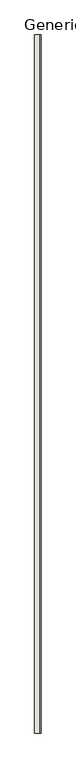
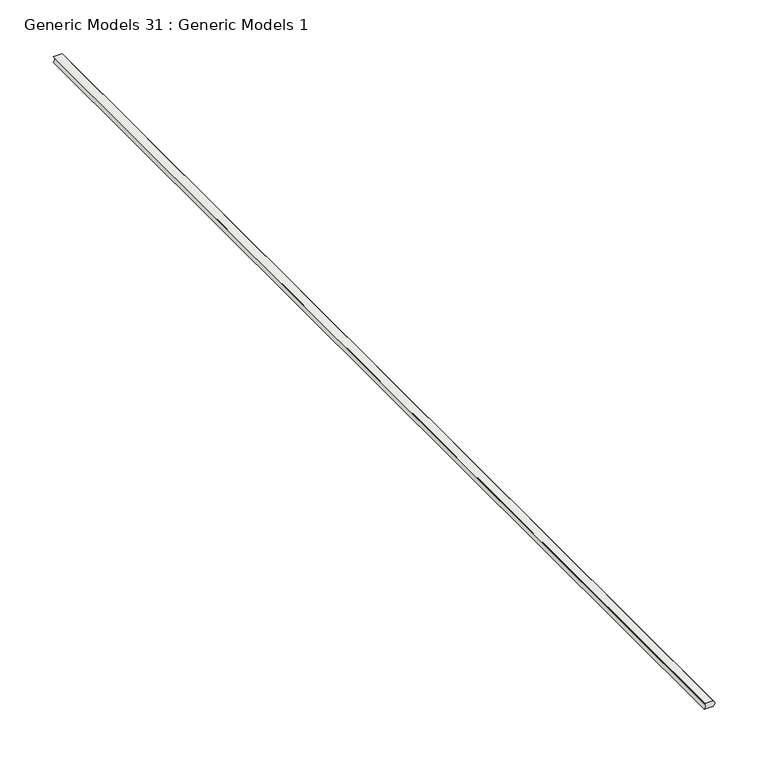
"""IFC4 building model written with IfcOpenShell, lengths in millimetres: wall geometry, Generic Models 31 : Generic Models 1."""

from ifc_helpers import new_model, si_unit, point, frame, frame_2d, origin, place, context, project, spatial, polyline, circle_curve, trimmed, segment, composite_curve, outline, extrude, source, transform, mapped, element, save


def generic_models_31_generic_models_1_7cb056b2(model_context):
    return source(origin(), model_context, "Body", "SweptSolid", [
        extrude(outline(composite_curve([segment(polyline([(0.0, 141116.05), (0.0, 141125.575)]), True, "CONTINUOUS"), segment(trimmed(circle_curve(frame_2d((3.175, 141122.6602595)), 4.3100275), [point((0.0, 141125.575))], [point((6.35, 141125.575))], False, "CARTESIAN"), True, "CONTINUOUS"), segment(polyline([(6.35, 141125.575), (6.35, 141116.05)]), True, "CONTINUOUS"), segment(trimmed(circle_curve(frame_2d((3.175, 141113.1352595)), 4.3100275), [point((6.35, 141116.05))], [point((0.0, 141116.05))], True, "CARTESIAN"), True, "CONTINUOUS")], self_intersect=False)), frame((0.0, 0.0, 0.0), z_axis=(0.0, 1.0, 0.0), x_axis=(0.0, 0.0, 1.0)), (0.0, 0.0, 1.0), 1219.2),
    ])


if __name__ == "__main__":
    model = new_model("IFC4")
    model_context = context("Model", 3, world=origin())
    ifc_project = project(units=[si_unit("LENGTHUNIT", "METRE", prefix="MILLI")], contexts=[model_context])
    site = spatial("IfcSite", under=ifc_project)
    building = spatial("IfcBuilding", under=site)
    placement = place(None, origin())
    generic_models_31_generic_models_1_shape = generic_models_31_generic_models_1_7cb056b2(model_context)
    element("IfcWall", 1, ObjectType="Generic Models 31 : Generic Models 1", at=placement, inside=building, context=model_context, shape_type="MappedRepresentation", body=[
        mapped(generic_models_31_generic_models_1_shape, transform((0.0, 0.0, 0.0), x_axis=(1.0, 0.0, 0.0), y_axis=(0.0, 1.0, 0.0), z_axis=(0.0, 0.0, 1.0))),
    ])
    save(model, "model.ifc")

# Revit data of these elements
# Element 1 (IfcWall, "Generic Models 31 : Generic Models 1")
#   Materials on its faces: "ACOUSTICAL SEALANT OR FIRE SEALANT, IF RATED WALL"
# Materials
#   "ACOUSTICAL SEALANT OR FIRE SEALANT, IF RATED WALL": class "Unassigned", colour RGB 120 120 120, transparency 0, Cost = 0
